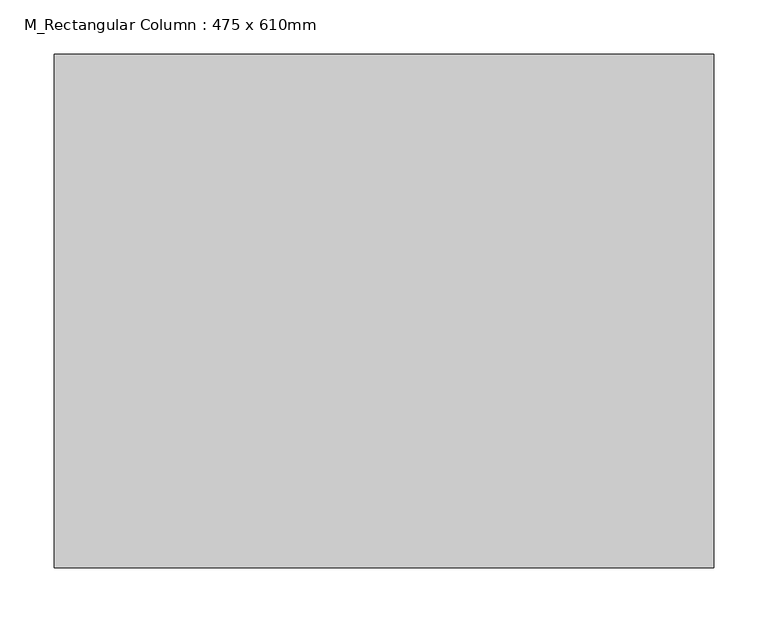
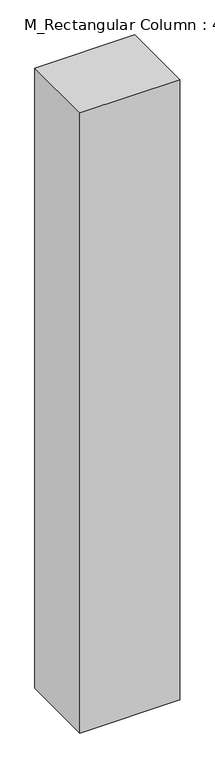
"""IFC4 building model written with IfcOpenShell, lengths in millimetres: column geometry, M_Rectangular Column : 475 x 610mm."""

from ifc_helpers import new_model, si_unit, origin, origin_with_axes, place, context, project, spatial, polyline, outline, extrude, source, transform, mapped, element, save


def m_rectangular_column_475_x_610mm_b7c60445(model_context):
    return source(origin(), model_context, "Body", "SweptSolid", [
        extrude(outline(polyline([(305.0, 237.5), (305.0, -237.5), (-305.0, -237.5), (-305.0, 237.5), (305.0, 237.5)])), origin_with_axes(), (0.0, 0.0, 1.0), 4000.0),
    ])


if __name__ == "__main__":
    model = new_model("IFC4")
    model_context = context("Model", 3, world=origin())
    ifc_project = project(units=[si_unit("LENGTHUNIT", "METRE", prefix="MILLI")], contexts=[model_context])
    site = spatial("IfcSite", under=ifc_project)
    building = spatial("IfcBuilding", under=site)
    placement = place(None, origin())
    m_rectangular_column_475_x_610mm_shape = m_rectangular_column_475_x_610mm_b7c60445(model_context)
    element("IfcColumn", 1, ObjectType="M_Rectangular Column : 475 x 610mm", at=placement, inside=building, context=model_context, shape_type="MappedRepresentation", body=[
        mapped(m_rectangular_column_475_x_610mm_shape, transform((0.0, 0.0, 0.0), x_axis=(1.0, 0.0, 0.0), y_axis=(0.0, 1.0, 0.0), z_axis=(0.0, 0.0, 1.0))),
    ])
    save(model, "model.ifc")

# Revit data of these elements
# Type "M_Rectangular Column : 475 x 610mm"
#   Depth = 475 mm
#   Offset Base = 0 mm
#   Offset Top = 0 mm
#   Width = 610 mm
#   Material = Copper
# Element 1 (IfcColumn, "M_Rectangular Column : 475 x 610mm")
#   Materials on its faces: "Copper"
# Materials
#   "Copper": class "Metal", colour RGB 0 0 0, transparency 0, Description = "Copper, matte finish", Cost = 0
